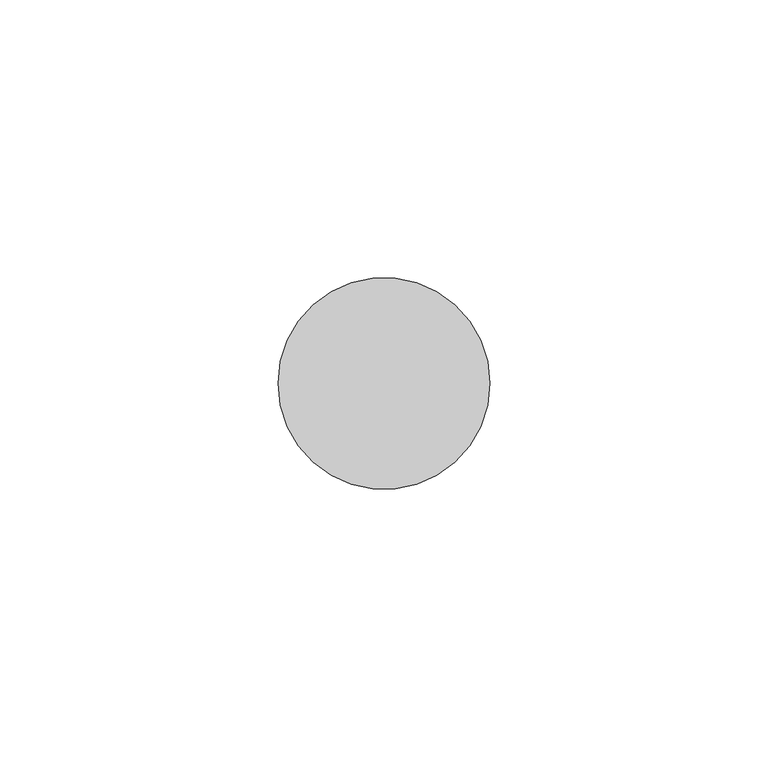
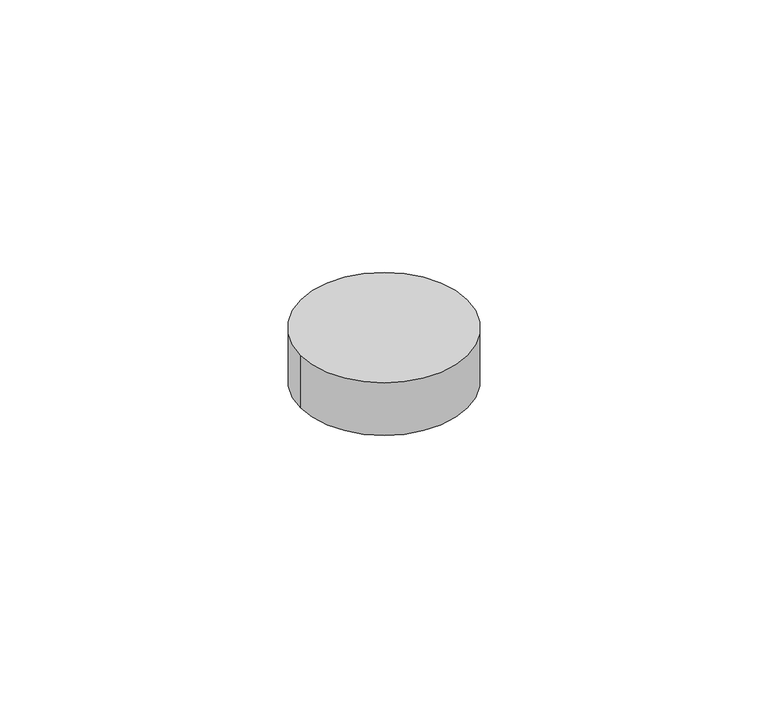
"""IFC4 building model written with IfcOpenShell, lengths in millimetres: proxy geometry, Bolt5:Bolt002:302951 : Bolt5:Bolt002:302951."""

import ifcopenshell
import ifcopenshell.guid

model = None  # the IFC model being written
_history = None  # IfcOwnerHistory: only IFC2X3 demands one
_inside = {}  # id of a spatial element -> (the spatial element, [elements in it])
_under = {}  # id of a project, library or spatial element -> (it, [spatial elements below it])
_declared = {}  # id of a project -> (the project, [libraries it declares])
_typed = {}  # id of a type object -> (the type object, [elements of that type])
_made_of = {}  # id of a material, layer set ... -> (it, [elements and type objects made of it])


def new_model(schema):
    """Start an empty IFC model of exactly this schema.

    Asked for "IFC4X3", IfcOpenShell would pick the latest addendum, in which some entities
    have other attributes; the version numbers below select the first issue.
    IFC2X3 requires an IfcOwnerHistory on every rooted entity: one is made here for all.
    """
    global model, _history
    if schema == "IFC4X3":
        model = ifcopenshell.file(schema_version=(4, 3, 0, 0))
    else:
        model = ifcopenshell.file(schema=schema)
    _inside.clear()
    _under.clear()
    _declared.clear()
    _typed.clear()
    _made_of.clear()
    _history = None
    if model.schema == "IFC2X3":
        org = make("IfcOrganization", Name="unknown")
        user = make(
            "IfcPersonAndOrganization",
            ThePerson=make("IfcPerson", FamilyName="unknown"),
            TheOrganization=org,
        )
        app = make(
            "IfcApplication",
            ApplicationDeveloper=org,
            Version="unknown",
            ApplicationFullName="unknown",
            ApplicationIdentifier="unknown",
        )
        _history = make(
            "IfcOwnerHistory",
            OwningUser=user,
            OwningApplication=app,
            ChangeAction="ADDED",
            CreationDate=0,
        )
    return model


def make(cls, **values):
    """One entity of the class cls with the attributes given. An attribute that is None is left unset."""
    return model.create_entity(
        cls, **{name: value for name, value in values.items() if value is not None}
    )


def rooted(cls, **values):
    """An entity with a GlobalId (a new one), such as an element, a storey or a relation."""
    return make(cls, GlobalId=ifcopenshell.guid.new(), OwnerHistory=_history, **values)


def si_unit(unit_type, name, prefix=None):
    """IfcSIUnit, for example si_unit("LENGTHUNIT", "METRE", prefix="MILLI")."""
    return make("IfcSIUnit", UnitType=unit_type, Prefix=prefix, Name=name)


def assignment(units):
    """IfcUnitAssignment: the units of a project."""
    return None if units is None else make("IfcUnitAssignment", Units=units)


def point(xyz):
    """IfcCartesianPoint."""
    return None if xyz is None else make("IfcCartesianPoint", Coordinates=xyz)


def direction(xyz):
    """IfcDirection."""
    return None if xyz is None else make("IfcDirection", DirectionRatios=xyz)


def frame(location, z_axis=None, x_axis=None):
    """IfcAxis2Placement3D, a coordinate frame: its origin and axes. An axis left out is left unset."""
    return make(
        "IfcAxis2Placement3D",
        Location=point(location),
        Axis=direction(z_axis),
        RefDirection=direction(x_axis),
    )


def frame_2d(location, x_axis=None):
    """IfcAxis2Placement2D, a coordinate frame in the plane: its origin and x axis."""
    return make(
        "IfcAxis2Placement2D", Location=point(location), RefDirection=direction(x_axis)
    )


def origin():
    """The frame at (0, 0, 0) with its axes left unset."""
    return frame((0.0, 0.0, 0.0))


def place(relative_to, where):
    """IfcLocalPlacement: puts the frame where relative to a parent placement (None: the world)."""
    return make(
        "IfcLocalPlacement", PlacementRelTo=relative_to, RelativePlacement=where
    )


def context(
    kind, dimensions, precision=None, world=None, true_north=None, identifier=None
):
    """IfcGeometricRepresentationContext, for example the 3D "Model" context."""
    return make(
        "IfcGeometricRepresentationContext",
        ContextIdentifier=identifier,
        ContextType=kind,
        CoordinateSpaceDimension=dimensions,
        Precision=precision,
        WorldCoordinateSystem=world,
        TrueNorth=true_north,
    )


def project(units=None, contexts=None):
    """IfcProject with its units and contexts."""
    return rooted(
        "IfcProject",
        Name="project",
        RepresentationContexts=contexts,
        UnitsInContext=assignment(units),
    )


def spatial(cls, under=None, at=None, **own):
    """A site, building, storey or space (cls), placed at a placement, below another one or the project."""
    s = rooted(cls, ObjectPlacement=at, **own)
    if under is not None:
        _under.setdefault(under.id(), (under, []))[1].append(s)
    return s


def circle_curve(where, radius):
    """IfcCircle in the frame where."""
    return make("IfcCircle", Position=where, Radius=radius)


def trimmed(basis, trim1, trim2, sense, master):
    """IfcTrimmedCurve: the piece of a basis curve between two trims."""
    return make(
        "IfcTrimmedCurve",
        BasisCurve=basis,
        Trim1=trim1,
        Trim2=trim2,
        SenseAgreement=sense,
        MasterRepresentation=master,
    )


def segment(curve, same_sense, transition):
    """IfcCompositeCurveSegment."""
    return make(
        "IfcCompositeCurveSegment",
        Transition=transition,
        SameSense=same_sense,
        ParentCurve=curve,
    )


def composite_curve(segments, self_intersect=None):
    """IfcCompositeCurve: segments joined end to end."""
    return make("IfcCompositeCurve", Segments=segments, SelfIntersect=self_intersect)


def outline(outer, holes=None, kind="AREA"):
    """IfcArbitraryClosedProfileDef: a profile drawn as a closed curve; with holes, ...WithVoids."""
    if holes is None:
        return make("IfcArbitraryClosedProfileDef", ProfileType=kind, OuterCurve=outer)
    return make(
        "IfcArbitraryProfileDefWithVoids",
        ProfileType=kind,
        OuterCurve=outer,
        InnerCurves=holes,
    )


def extrude(swept, where, along, depth):
    """IfcExtrudedAreaSolid: the profile swept, set in the frame where, extruded along a direction by depth."""
    return make(
        "IfcExtrudedAreaSolid",
        SweptArea=swept,
        Position=where,
        ExtrudedDirection=direction(along),
        Depth=depth,
    )


def shape(context_of_items, identifier, shape_type, items):
    """IfcShapeRepresentation: the items that make up one representation, for example the "Body"."""
    return make(
        "IfcShapeRepresentation",
        ContextOfItems=context_of_items,
        RepresentationIdentifier=identifier,
        RepresentationType=shape_type,
        Items=items,
    )


def source(mapping_origin, context_of_items, identifier, shape_type, items):
    """IfcRepresentationMap: a shape defined once, which mapped items show again and again."""
    return make(
        "IfcRepresentationMap",
        MappingOrigin=mapping_origin,
        MappedRepresentation=shape(context_of_items, identifier, shape_type, items),
    )


def transform(
    local_origin,
    x_axis=None,
    y_axis=None,
    z_axis=None,
    scale=None,
    scale2=None,
    scale3=None,
    uniform=True,
):
    """IfcCartesianTransformationOperator3D, or its non-uniform kind. x_axis, y_axis, z_axis: its Axis1, 2, 3."""
    if uniform:
        return make(
            "IfcCartesianTransformationOperator3D",
            Axis1=direction(x_axis),
            Axis2=direction(y_axis),
            LocalOrigin=point(local_origin),
            Scale=scale,
            Axis3=direction(z_axis),
        )
    return make(
        "IfcCartesianTransformationOperator3DnonUniform",
        Axis1=direction(x_axis),
        Axis2=direction(y_axis),
        LocalOrigin=point(local_origin),
        Scale=scale,
        Axis3=direction(z_axis),
        Scale2=scale2,
        Scale3=scale3,
    )


def mapped(mapping_source, mapping_target):
    """IfcMappedItem: shows the shape of a source again, moved by a transform."""
    return make(
        "IfcMappedItem", MappingSource=mapping_source, MappingTarget=mapping_target
    )


def made_of(thing, what):
    """Note that an element or type object is made of a material, layer set ...; save() writes the relation."""
    if what is not None:
        _made_of.setdefault(what.id(), (what, []))[1].append(thing)
    return thing


def element(
    cls,
    number,
    at=None,
    inside=None,
    cuts=None,
    type_object=None,
    material=None,
    context=None,
    identifier="Body",
    shape_type=None,
    held_by="IfcProductDefinitionShape",
    body=None,
    shapes=None,
    **own,
):
    """One element of the class cls, such as IfcWall. Its Tag is "e" and its number.

    at: its placement. inside: the storey or other place that contains it. cuts: it is an
    opening in that element (IfcRelVoidsElement). A single representation is given by context,
    identifier, shape_type and body (its items); several are given by shapes. held_by: the class
    of the entity that holds the representations. save() writes the other relations.
    """
    e = rooted(cls, Tag="e%d" % number, ObjectPlacement=at, **own)
    if body is not None:
        shapes = [shape(context, identifier, shape_type, body)]
    if shapes is not None:
        e.Representation = make(held_by, Representations=shapes)
    if inside is not None:
        _inside.setdefault(inside.id(), (inside, []))[1].append(e)
    if cuts is not None:
        rooted(
            "IfcRelVoidsElement", RelatingBuildingElement=cuts, RelatedOpeningElement=e
        )
    if type_object is not None:
        _typed.setdefault(type_object.id(), (type_object, []))[1].append(e)
    return made_of(e, material)


def aggregate(whole, parts):
    """IfcRelAggregates: a whole, such as a stair, and the parts it consists of."""
    return rooted("IfcRelAggregates", RelatingObject=whole, RelatedObjects=parts)


def save(model, path):
    """Write the relations noted so far, then the file.

    IfcRelAggregates (storeys below a building ...), IfcRelContainedInSpatialStructure (elements
    in a storey), IfcRelDefinesByType, IfcRelAssociatesMaterial and IfcRelDeclares: one each for
    every whole, place, type object, material and project.
    """
    for whole, parts in _under.values():
        aggregate(whole, parts)
    for where, things in _inside.values():
        rooted(
            "IfcRelContainedInSpatialStructure",
            RelatedElements=things,
            RelatingStructure=where,
        )
    for kind, things in _typed.values():
        rooted("IfcRelDefinesByType", RelatedObjects=things, RelatingType=kind)
    for what, things in _made_of.values():
        rooted("IfcRelAssociatesMaterial", RelatedObjects=things, RelatingMaterial=what)
    for by, libraries in _declared.values():
        rooted("IfcRelDeclares", RelatingContext=by, RelatedDefinitions=libraries)
    model.write(path)


def generic_models_6da721b0(model_context):
    return source(origin(), model_context, "Body", "SweptSolid", [
        extrude(outline(composite_curve([segment(trimmed(circle_curve(frame_2d((12192.2703385, -1503.5124296)), 19.05), [point((12173.2203385, -1503.5124296))], [point((12211.3203385, -1503.5124296))], False, "CARTESIAN"), True, "CONTINUOUS"), segment(trimmed(circle_curve(frame_2d((12192.2703385, -1503.5124296)), 19.05), [point((12211.3203385, -1503.5124296))], [point((12173.2203385, -1503.5124296))], False, "CARTESIAN"), True, "CONTINUOUS")], self_intersect=False)), frame((0.0, 0.0, 40068.246), z_axis=(0.0, 0.0, 1.0), x_axis=(1.0, 0.0, 0.0)), (0.0, 0.0, 1.0), 12.7),
    ])


if __name__ == "__main__":
    model = new_model("IFC4")
    model_context = context("Model", 3, world=origin())
    ifc_project = project(units=[si_unit("LENGTHUNIT", "METRE", prefix="MILLI")], contexts=[model_context])
    site = spatial("IfcSite", under=ifc_project)
    building = spatial("IfcBuilding", under=site)
    placement = place(None, origin())
    generic_models_shape = generic_models_6da721b0(model_context)
    element("IfcBuildingElementProxy", 1, Name="Bolt5:Bolt002:302951 : Bolt5:Bolt002:302951", ObjectType="Bolt5:Bolt002:302951 : Bolt5:Bolt002:302951", at=placement, inside=building, context=model_context, shape_type="MappedRepresentation", body=[
        mapped(generic_models_shape, transform((0.0, 0.0, 0.0), x_axis=(1.0, 0.0, 0.0), y_axis=(0.0, 1.0, 0.0), z_axis=(0.0, 0.0, 1.0))),
    ])
    save(model, "model.ifc")

# Revit data of these elements
# Type "Bolt5:Bolt002:302951 : Bolt5:Bolt002:302951"
#   NameOverride = "Bolt5:Bolt002:302951"
#   ObjectTypeOverride = "Bolt5:Bolt002"
#   Reference = "Bolt002"
#   Category = "Generic Models"
#   Tag = "302951"
# Element 1 (IfcBuildingElementProxy, "Bolt5:Bolt002:302951 : Bolt5:Bolt002:302951")
#   Materials on its faces: "BOLTS CONCEALED BY FLOOR FINISH"
# Materials
#   "BOLTS CONCEALED BY FLOOR FINISH": class "Unassigned", colour RGB 128 128 128, transparency 0
